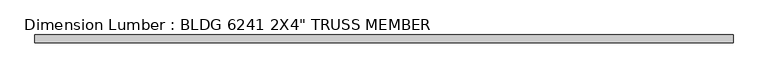
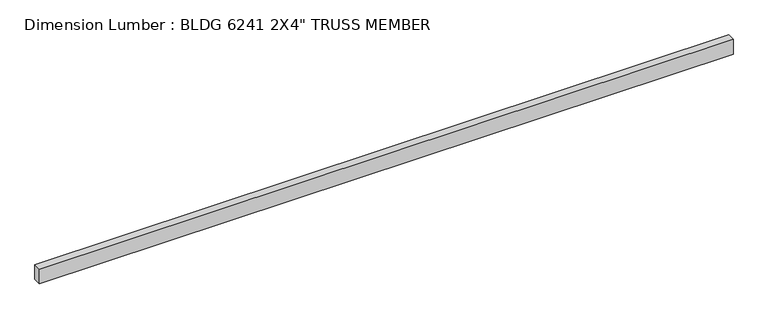
"""IFC4 building model written with IfcOpenShell, lengths in millimetres: beam geometry."""

from ifc_helpers import new_model, si_unit, frame, origin, place, context, project, spatial, polyline, outline, extrude, source, transform, mapped, element, save


def beam_175a3536(model_context):
    return source(origin(), model_context, "Body", "SweptSolid", [
        extrude(outline(polyline([(2249.4875, 25.4), (2249.4875, -25.4), (-2249.4874994, -25.4), (-2249.4874994, 25.4), (2249.4875, 25.4)])), frame((0.0, 0.0, -50.8), z_axis=(0.0, 0.0, 1.0), x_axis=(1.0, 0.0, 0.0)), (0.0, 0.0, 1.0), 101.6),
    ])


if __name__ == "__main__":
    model = new_model("IFC4")
    model_context = context("Model", 3, world=origin())
    ifc_project = project(units=[si_unit("LENGTHUNIT", "METRE", prefix="MILLI")], contexts=[model_context])
    site = spatial("IfcSite", under=ifc_project)
    building = spatial("IfcBuilding", under=site)
    placement = place(None, origin())
    beam_shape = beam_175a3536(model_context)
    element("IfcBeam", 1, ObjectType="Dimension Lumber : BLDG 6241 2X4\" TRUSS MEMBER", at=placement, inside=building, context=model_context, shape_type="MappedRepresentation", body=[
        mapped(beam_shape, transform((0.0, 0.0, 0.0), x_axis=(1.0, 0.0, 0.0), y_axis=(0.0, 1.0, 0.0), z_axis=(0.0, 0.0, 1.0))),
    ])
    save(model, "model.ifc")

# Revit data of these elements
# Type "Dimension Lumber : BLDG 6241 2X4\" TRUSS MEMBER"
#   Assembly Code = "B10"
#   A = 0.273472 SF
#   Length [instance default] = 5' - 0"
#   b = 0' - 2"
#   d = 0' - 4"
#   Structural Material [instance default] = Softwood, Lumber
# Element 1 (IfcBeam, "Dimension Lumber : BLDG 6241 2X4\" TRUSS MEMBER")
#   Materials on its faces: "Softwood, Lumber"
# Materials
#   "Softwood, Lumber": class "Wood", colour RGB 223 192 134, transparency 0, Description = "Pinus Echinata", Cost = 0
